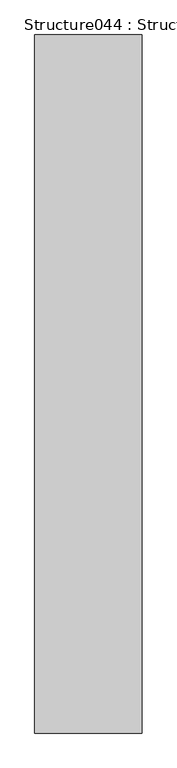
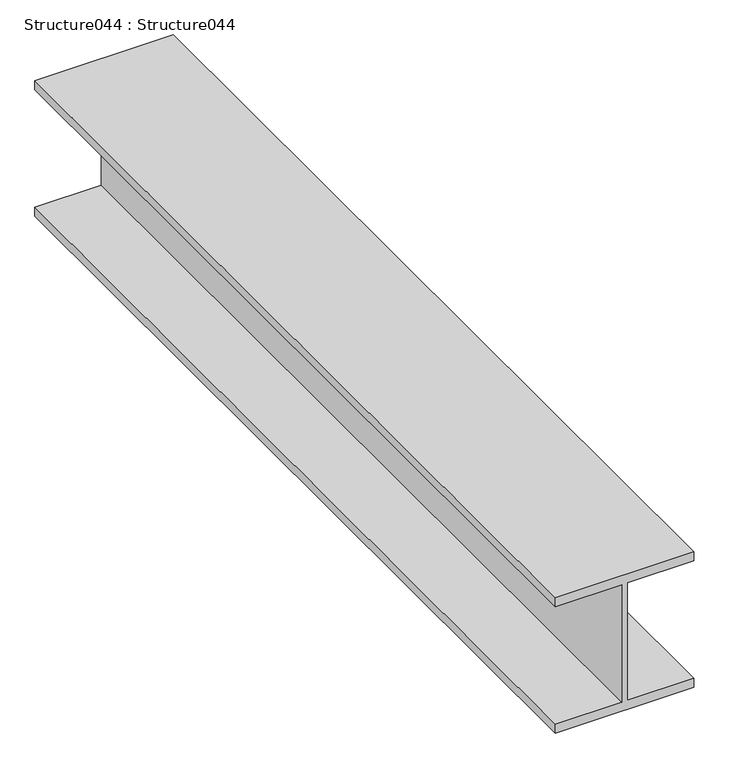
"""IFC4 building model written with IfcOpenShell, lengths in millimetres: proxy geometry, Structure044 : Structure044."""

from ifc_helpers import new_model, si_unit, frame, origin, place, context, project, spatial, polyline, outline, extrude, source, transform, mapped, element, save


def structure044_structure044_d6db8104(model_context):
    return source(origin(), model_context, "Body", "SweptSolid", [
        extrude(outline(polyline([(40092.122, -1049.2769422), (39815.77, -1049.2769422), (39815.77, -1196.4064422), (39795.196, -1196.4064422), (39795.196, -889.0664422), (39815.77, -889.0664422), (39815.77, -1036.1959422), (40092.122, -1036.1959422), (40092.122, -889.0664422), (40112.696, -889.0664422), (40112.696, -1196.4064422), (40092.122, -1196.4064422), (40092.122, -1049.2769422)])), frame((0.0, -1052.8906574, 0.0), z_axis=(0.0, 1.0, 0.0), x_axis=(0.0, 0.0, 1.0)), (0.0, 0.0, 1.0), 2000.0),
    ])


if __name__ == "__main__":
    model = new_model("IFC4")
    model_context = context("Model", 3, world=origin())
    ifc_project = project(units=[si_unit("LENGTHUNIT", "METRE", prefix="MILLI")], contexts=[model_context])
    site = spatial("IfcSite", under=ifc_project)
    building = spatial("IfcBuilding", under=site)
    placement = place(None, origin())
    structure044_structure044_shape = structure044_structure044_d6db8104(model_context)
    element("IfcBuildingElementProxy", 1, Name="Structure044 : Structure044", ObjectType="Structure044 : Structure044", at=placement, inside=building, context=model_context, shape_type="MappedRepresentation", body=[
        mapped(structure044_structure044_shape, transform((0.0, 0.0, 0.0), x_axis=(1.0, 0.0, 0.0), y_axis=(0.0, 1.0, 0.0), z_axis=(0.0, 0.0, 1.0))),
    ])
    save(model, "model.ifc")

# Revit data of these elements
# Type "Structure044 : Structure044"
#   NameOverride = "Structure044"
# Element 1 (IfcBuildingElementProxy, "Structure044 : Structure044")
#   Materials on its faces: "METAL STRUCTURE (SEE STRUCTURAL DWGS)"
# Materials
#   "METAL STRUCTURE (SEE STRUCTURAL DWGS)": class "Unassigned", colour RGB 128 128 128, transparency 0
